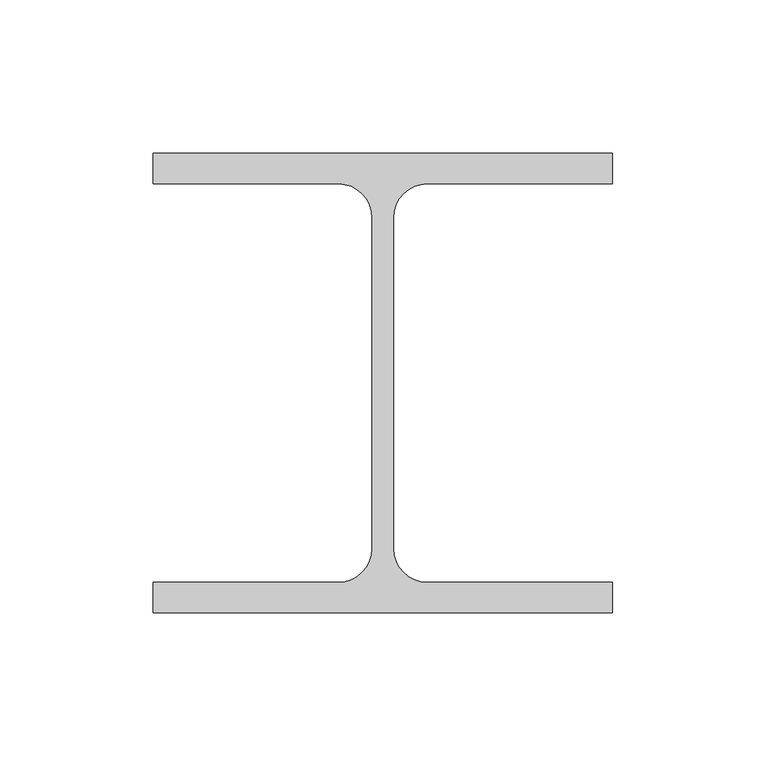
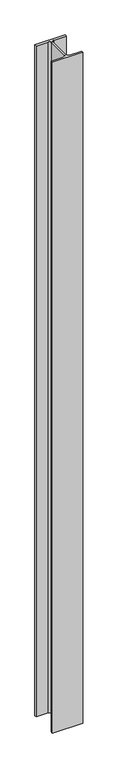
"""IFC4 building model written with IfcOpenShell, lengths in millimetres: column geometry, 0912_Steel Column_H_KSD3502 : H_SC_ASC_H-150x150x7x10."""

from ifc_helpers import new_model, si_unit, point, frame, frame_2d, origin, place, context, project, spatial, polyline, circle_curve, trimmed, segment, composite_curve, outline, extrude, source, transform, mapped, element, save


def column_aafab9da(model_context):
    return source(origin(), model_context, "Body", "SweptSolid", [
        extrude(outline(composite_curve([segment(polyline([(75.0, 75.0), (75.0, 65.0), (14.5, 65.0)]), True, "CONTINUOUS"), segment(trimmed(circle_curve(frame_2d((14.5, 54.0)), 11.0), [point((14.5, 65.0))], [point((3.5, 54.0))], True, "CARTESIAN"), True, "CONTINUOUS"), segment(polyline([(3.5, 54.0), (3.5, -54.0)]), True, "CONTINUOUS"), segment(trimmed(circle_curve(frame_2d((14.5, -54.0)), 11.0), [point((3.5, -54.0))], [point((14.5, -65.0))], True, "CARTESIAN"), True, "CONTINUOUS"), segment(polyline([(14.5, -65.0), (75.0, -65.0), (75.0, -75.0), (-75.0, -75.0), (-75.0, -65.0), (-14.5, -65.0)]), True, "CONTINUOUS"), segment(trimmed(circle_curve(frame_2d((-14.5, -54.0)), 11.0), [point((-14.5, -65.0))], [point((-3.5, -54.0))], True, "CARTESIAN"), True, "CONTINUOUS"), segment(polyline([(-3.5, -54.0), (-3.5, 54.0)]), True, "CONTINUOUS"), segment(trimmed(circle_curve(frame_2d((-14.5, 54.0)), 11.0), [point((-3.5, 54.0))], [point((-14.5, 65.0))], True, "CARTESIAN"), True, "CONTINUOUS"), segment(polyline([(-14.5, 65.0), (-75.0, 65.0), (-75.0, 75.0), (75.0, 75.0)]), True, "CONTINUOUS")], self_intersect=False)), frame((0.0, 0.0, 4449.9720055), z_axis=(0.0, 0.0, 1.0), x_axis=(1.0, 0.0, 0.0)), (0.0, 0.0, 1.0), 3510.0),
    ])


if __name__ == "__main__":
    model = new_model("IFC4")
    model_context = context("Model", 3, world=origin())
    ifc_project = project(units=[si_unit("LENGTHUNIT", "METRE", prefix="MILLI")], contexts=[model_context])
    site = spatial("IfcSite", under=ifc_project)
    building = spatial("IfcBuilding", under=site)
    placement = place(None, origin())
    column_shape = column_aafab9da(model_context)
    element("IfcColumn", 1, ObjectType="0912_Steel Column_H_KSD3502 : H_SC_ASC_H-150x150x7x10", at=placement, inside=building, context=model_context, shape_type="MappedRepresentation", body=[
        mapped(column_shape, transform((0.0, 0.0, 0.0), x_axis=(1.0, 0.0, 0.0), y_axis=(0.0, 1.0, 0.0), z_axis=(0.0, 0.0, 1.0))),
    ])
    save(model, "model.ifc")

# Revit data of these elements
# Type "0912_Steel Column_H_KSD3502 : H_SC_ASC_H-150x150x7x10"
#   H_WM Code_1 = "S01AA002-00001 | Main Steel Structure Fabrication Work | Shelter/Building | Medium Steel - Standard (90KG/M>Weight≥30KG/M) | Material: (   )"
#   H_WM Code_2 = "S03AA028-00001 | Main Steel Structure Erection Work | Shelter/Building | Medium Steel (90KG/M>Weight≥30KG/M) | Material: (   )"
#   H_WM Code_3 = "S01AA010-00001 | Main Steel Structure Fabrication Work | Shelter/Building | Steel Painting/Coating | for Non-Fireproofed Steel Surface, Surface Preparation, Primer, Second & Final Coat | Material: (   )"
#   H_Q'ty Cal Type Tag = "SC-Q2"
#   Width = 15.0 cm
#   Web Thickness = 0.7 cm
#   Web Fillet = 1.1 cm
#   Warping Constant = 27562.5 cm⁶
#   Torsional Moment of Inertia = 11.6007 cm⁴
#   Section Area = 40.14 cm²
#   Plastic Modulus weak axis = 115.0 cm³
#   Plastic Modulus strong axis = 246.0 cm³
#   Perimeter = 0.87 m²/m
#   Nominal Weight = 31.50 kgf/m
#   Moment of Inertia weak axis = 563.00 cm⁴
#   Moment of Inertia strong axis = 1640.00 cm⁴
#   Height = 15.0 cm
#   Flange Thickness = 1.0 cm
#   Elastic Modulus weak axis = 75.1 cm³
#   Elastic Modulus strong axis = 219.0 cm³
#   Centroid Vertical = 7.5 cm
#   Centroid Horizontal = 7.5 cm
#   Structural Material [instance default] = Steel, 45-345
#   Section Name Key = ""
#   Bolt Spacing = 0
#   Assembly Code = ""
# Element 1 (IfcColumn, "0912_Steel Column_H_KSD3502 : H_SC_ASC_H-150x150x7x10")
#   Structural Material = none
# Materials
#   "Steel, 45-345": class "Metal", colour RGB 189 187 185, transparency 0, Description = "Steel 345 MPa", Cost = 0
